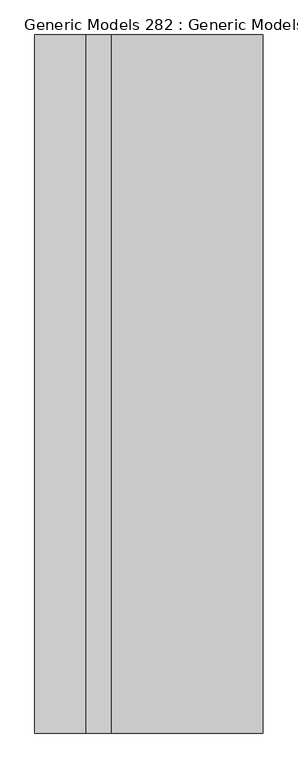
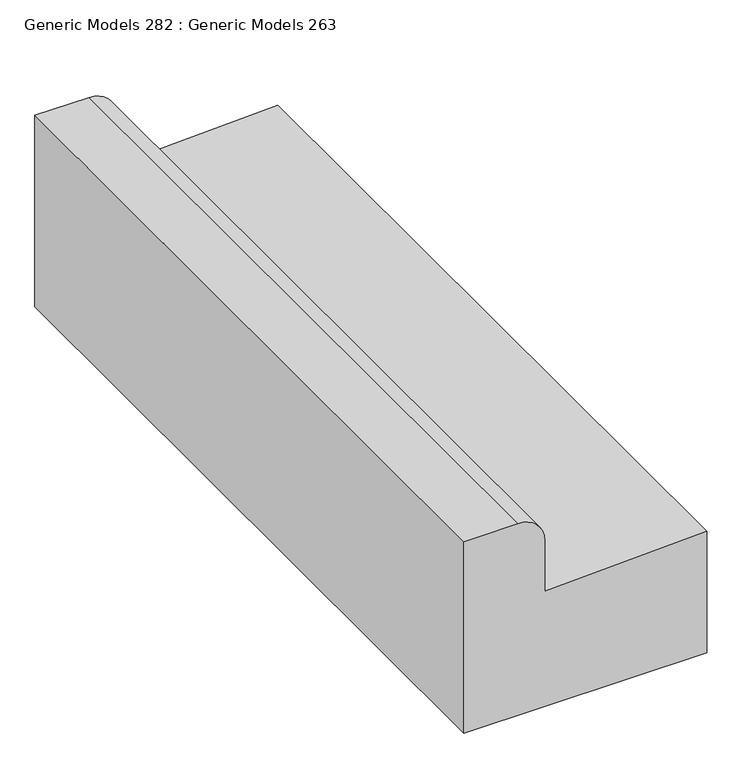
"""IFC4 building model written with IfcOpenShell, lengths in millimetres: proxy geometry, Generic Models 282 : Generic Models 263."""

import ifcopenshell
import ifcopenshell.guid

model = None  # the IFC model being written
_history = None  # IfcOwnerHistory: only IFC2X3 demands one
_inside = {}  # id of a spatial element -> (the spatial element, [elements in it])
_under = {}  # id of a project, library or spatial element -> (it, [spatial elements below it])
_declared = {}  # id of a project -> (the project, [libraries it declares])
_typed = {}  # id of a type object -> (the type object, [elements of that type])
_made_of = {}  # id of a material, layer set ... -> (it, [elements and type objects made of it])


def new_model(schema):
    """Start an empty IFC model of exactly this schema.

    Asked for "IFC4X3", IfcOpenShell would pick the latest addendum, in which some entities
    have other attributes; the version numbers below select the first issue.
    IFC2X3 requires an IfcOwnerHistory on every rooted entity: one is made here for all.
    """
    global model, _history
    if schema == "IFC4X3":
        model = ifcopenshell.file(schema_version=(4, 3, 0, 0))
    else:
        model = ifcopenshell.file(schema=schema)
    _inside.clear()
    _under.clear()
    _declared.clear()
    _typed.clear()
    _made_of.clear()
    _history = None
    if model.schema == "IFC2X3":
        org = make("IfcOrganization", Name="unknown")
        user = make(
            "IfcPersonAndOrganization",
            ThePerson=make("IfcPerson", FamilyName="unknown"),
            TheOrganization=org,
        )
        app = make(
            "IfcApplication",
            ApplicationDeveloper=org,
            Version="unknown",
            ApplicationFullName="unknown",
            ApplicationIdentifier="unknown",
        )
        _history = make(
            "IfcOwnerHistory",
            OwningUser=user,
            OwningApplication=app,
            ChangeAction="ADDED",
            CreationDate=0,
        )
    return model


def make(cls, **values):
    """One entity of the class cls with the attributes given. An attribute that is None is left unset."""
    return model.create_entity(
        cls, **{name: value for name, value in values.items() if value is not None}
    )


def rooted(cls, **values):
    """An entity with a GlobalId (a new one), such as an element, a storey or a relation."""
    return make(cls, GlobalId=ifcopenshell.guid.new(), OwnerHistory=_history, **values)


def si_unit(unit_type, name, prefix=None):
    """IfcSIUnit, for example si_unit("LENGTHUNIT", "METRE", prefix="MILLI")."""
    return make("IfcSIUnit", UnitType=unit_type, Prefix=prefix, Name=name)


def assignment(units):
    """IfcUnitAssignment: the units of a project."""
    return None if units is None else make("IfcUnitAssignment", Units=units)


def point(xyz):
    """IfcCartesianPoint."""
    return None if xyz is None else make("IfcCartesianPoint", Coordinates=xyz)


def direction(xyz):
    """IfcDirection."""
    return None if xyz is None else make("IfcDirection", DirectionRatios=xyz)


def frame(location, z_axis=None, x_axis=None):
    """IfcAxis2Placement3D, a coordinate frame: its origin and axes. An axis left out is left unset."""
    return make(
        "IfcAxis2Placement3D",
        Location=point(location),
        Axis=direction(z_axis),
        RefDirection=direction(x_axis),
    )


def frame_2d(location, x_axis=None):
    """IfcAxis2Placement2D, a coordinate frame in the plane: its origin and x axis."""
    return make(
        "IfcAxis2Placement2D", Location=point(location), RefDirection=direction(x_axis)
    )


def origin():
    """The frame at (0, 0, 0) with its axes left unset."""
    return frame((0.0, 0.0, 0.0))


def place(relative_to, where):
    """IfcLocalPlacement: puts the frame where relative to a parent placement (None: the world)."""
    return make(
        "IfcLocalPlacement", PlacementRelTo=relative_to, RelativePlacement=where
    )


def context(
    kind, dimensions, precision=None, world=None, true_north=None, identifier=None
):
    """IfcGeometricRepresentationContext, for example the 3D "Model" context."""
    return make(
        "IfcGeometricRepresentationContext",
        ContextIdentifier=identifier,
        ContextType=kind,
        CoordinateSpaceDimension=dimensions,
        Precision=precision,
        WorldCoordinateSystem=world,
        TrueNorth=true_north,
    )


def project(units=None, contexts=None):
    """IfcProject with its units and contexts."""
    return rooted(
        "IfcProject",
        Name="project",
        RepresentationContexts=contexts,
        UnitsInContext=assignment(units),
    )


def spatial(cls, under=None, at=None, **own):
    """A site, building, storey or space (cls), placed at a placement, below another one or the project."""
    s = rooted(cls, ObjectPlacement=at, **own)
    if under is not None:
        _under.setdefault(under.id(), (under, []))[1].append(s)
    return s


def polyline(points):
    """IfcPolyline through the points."""
    return make("IfcPolyline", Points=[point(p) for p in points])


def circle_curve(where, radius):
    """IfcCircle in the frame where."""
    return make("IfcCircle", Position=where, Radius=radius)


def trimmed(basis, trim1, trim2, sense, master):
    """IfcTrimmedCurve: the piece of a basis curve between two trims."""
    return make(
        "IfcTrimmedCurve",
        BasisCurve=basis,
        Trim1=trim1,
        Trim2=trim2,
        SenseAgreement=sense,
        MasterRepresentation=master,
    )


def segment(curve, same_sense, transition):
    """IfcCompositeCurveSegment."""
    return make(
        "IfcCompositeCurveSegment",
        Transition=transition,
        SameSense=same_sense,
        ParentCurve=curve,
    )


def composite_curve(segments, self_intersect=None):
    """IfcCompositeCurve: segments joined end to end."""
    return make("IfcCompositeCurve", Segments=segments, SelfIntersect=self_intersect)


def outline(outer, holes=None, kind="AREA"):
    """IfcArbitraryClosedProfileDef: a profile drawn as a closed curve; with holes, ...WithVoids."""
    if holes is None:
        return make("IfcArbitraryClosedProfileDef", ProfileType=kind, OuterCurve=outer)
    return make(
        "IfcArbitraryProfileDefWithVoids",
        ProfileType=kind,
        OuterCurve=outer,
        InnerCurves=holes,
    )


def extrude(swept, where, along, depth):
    """IfcExtrudedAreaSolid: the profile swept, set in the frame where, extruded along a direction by depth."""
    return make(
        "IfcExtrudedAreaSolid",
        SweptArea=swept,
        Position=where,
        ExtrudedDirection=direction(along),
        Depth=depth,
    )


def shape(context_of_items, identifier, shape_type, items):
    """IfcShapeRepresentation: the items that make up one representation, for example the "Body"."""
    return make(
        "IfcShapeRepresentation",
        ContextOfItems=context_of_items,
        RepresentationIdentifier=identifier,
        RepresentationType=shape_type,
        Items=items,
    )


def source(mapping_origin, context_of_items, identifier, shape_type, items):
    """IfcRepresentationMap: a shape defined once, which mapped items show again and again."""
    return make(
        "IfcRepresentationMap",
        MappingOrigin=mapping_origin,
        MappedRepresentation=shape(context_of_items, identifier, shape_type, items),
    )


def transform(
    local_origin,
    x_axis=None,
    y_axis=None,
    z_axis=None,
    scale=None,
    scale2=None,
    scale3=None,
    uniform=True,
):
    """IfcCartesianTransformationOperator3D, or its non-uniform kind. x_axis, y_axis, z_axis: its Axis1, 2, 3."""
    if uniform:
        return make(
            "IfcCartesianTransformationOperator3D",
            Axis1=direction(x_axis),
            Axis2=direction(y_axis),
            LocalOrigin=point(local_origin),
            Scale=scale,
            Axis3=direction(z_axis),
        )
    return make(
        "IfcCartesianTransformationOperator3DnonUniform",
        Axis1=direction(x_axis),
        Axis2=direction(y_axis),
        LocalOrigin=point(local_origin),
        Scale=scale,
        Axis3=direction(z_axis),
        Scale2=scale2,
        Scale3=scale3,
    )


def mapped(mapping_source, mapping_target):
    """IfcMappedItem: shows the shape of a source again, moved by a transform."""
    return make(
        "IfcMappedItem", MappingSource=mapping_source, MappingTarget=mapping_target
    )


def made_of(thing, what):
    """Note that an element or type object is made of a material, layer set ...; save() writes the relation."""
    if what is not None:
        _made_of.setdefault(what.id(), (what, []))[1].append(thing)
    return thing


def element(
    cls,
    number,
    at=None,
    inside=None,
    cuts=None,
    type_object=None,
    material=None,
    context=None,
    identifier="Body",
    shape_type=None,
    held_by="IfcProductDefinitionShape",
    body=None,
    shapes=None,
    **own,
):
    """One element of the class cls, such as IfcWall. Its Tag is "e" and its number.

    at: its placement. inside: the storey or other place that contains it. cuts: it is an
    opening in that element (IfcRelVoidsElement). A single representation is given by context,
    identifier, shape_type and body (its items); several are given by shapes. held_by: the class
    of the entity that holds the representations. save() writes the other relations.
    """
    e = rooted(cls, Tag="e%d" % number, ObjectPlacement=at, **own)
    if body is not None:
        shapes = [shape(context, identifier, shape_type, body)]
    if shapes is not None:
        e.Representation = make(held_by, Representations=shapes)
    if inside is not None:
        _inside.setdefault(inside.id(), (inside, []))[1].append(e)
    if cuts is not None:
        rooted(
            "IfcRelVoidsElement", RelatingBuildingElement=cuts, RelatedOpeningElement=e
        )
    if type_object is not None:
        _typed.setdefault(type_object.id(), (type_object, []))[1].append(e)
    return made_of(e, material)


def aggregate(whole, parts):
    """IfcRelAggregates: a whole, such as a stair, and the parts it consists of."""
    return rooted("IfcRelAggregates", RelatingObject=whole, RelatedObjects=parts)


def save(model, path):
    """Write the relations noted so far, then the file.

    IfcRelAggregates (storeys below a building ...), IfcRelContainedInSpatialStructure (elements
    in a storey), IfcRelDefinesByType, IfcRelAssociatesMaterial and IfcRelDeclares: one each for
    every whole, place, type object, material and project.
    """
    for whole, parts in _under.values():
        aggregate(whole, parts)
    for where, things in _inside.values():
        rooted(
            "IfcRelContainedInSpatialStructure",
            RelatedElements=things,
            RelatingStructure=where,
        )
    for kind, things in _typed.values():
        rooted("IfcRelDefinesByType", RelatedObjects=things, RelatingType=kind)
    for what, things in _made_of.values():
        rooted("IfcRelAssociatesMaterial", RelatedObjects=things, RelatingMaterial=what)
    for by, libraries in _declared.values():
        rooted("IfcRelDeclares", RelatingContext=by, RelatedDefinitions=libraries)
    model.write(path)


def generic_models_282_generic_models_263_cc0d5e36(model_context):
    return source(origin(), model_context, "Body", "SweptSolid", [
        extrude(outline(composite_curve([segment(polyline([(0.0, 91681.5797726), (0.0, 91579.9797726), (-381.0, 91579.9797726), (-381.0, 92037.1797726), (-139.7, 92037.1797726), (-152.4, 91732.3797726), (-50.8, 91732.3797726)]), True, "CONTINUOUS"), segment(trimmed(circle_curve(frame_2d((-50.8, 91681.5797726)), 50.8), [point((-50.8, 91732.3797726))], [point((0.0, 91681.5797726))], False, "CARTESIAN"), True, "CONTINUOUS")], self_intersect=False)), frame((0.0, 2106.5727422, 0.0), z_axis=(0.0, 1.0, 0.0), x_axis=(0.0, 0.0, 1.0)), (0.0, 0.0, 1.0), 1397.4322547),
    ])


if __name__ == "__main__":
    model = new_model("IFC4")
    model_context = context("Model", 3, world=origin())
    ifc_project = project(units=[si_unit("LENGTHUNIT", "METRE", prefix="MILLI")], contexts=[model_context])
    site = spatial("IfcSite", under=ifc_project)
    building = spatial("IfcBuilding", under=site)
    placement = place(None, origin())
    generic_models_282_generic_models_263_shape = generic_models_282_generic_models_263_cc0d5e36(model_context)
    element("IfcBuildingElementProxy", 1, Name="Generic Models 282 : Generic Models 263", ObjectType="Generic Models 282 : Generic Models 263", at=placement, inside=building, context=model_context, shape_type="MappedRepresentation", body=[
        mapped(generic_models_282_generic_models_263_shape, transform((0.0, 0.0, 0.0), x_axis=(1.0, 0.0, 0.0), y_axis=(0.0, 1.0, 0.0), z_axis=(0.0, 0.0, 1.0))),
    ])
    save(model, "model.ifc")

# Revit data of these elements
# Element 1 (IfcBuildingElementProxy, "Generic Models 282 : Generic Models 263")
#   Materials on its faces: "CONCRETE CURB"
# Materials
#   "CONCRETE CURB": class "Concrete", colour RGB 191 191 191, transparency 0, Description = "Cast-in-place concrete", Cost = 0
